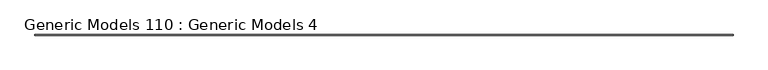
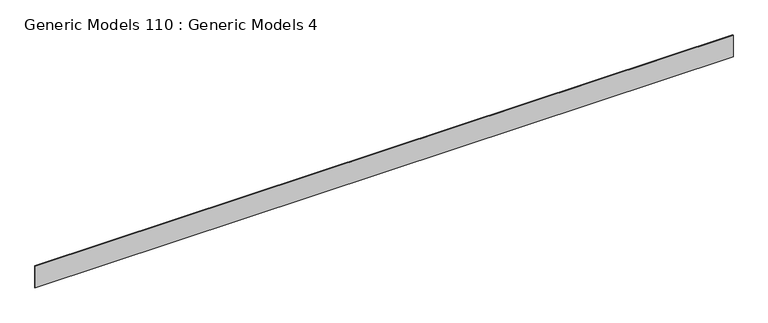
"""IFC4 building model written with IfcOpenShell, lengths in millimetres: proxy geometry, Generic Models 110 : Generic Models 4."""

from ifc_helpers import new_model, si_unit, frame, origin, place, context, project, spatial, polyline, outline, extrude, source, transform, mapped, element, save


def generic_models_110_generic_models_4_491da27e(model_context):
    return source(origin(), model_context, "Body", "SweptSolid", [
        extrude(outline(polyline([(8383.6828684, 7053.8569221), (8383.6828684, 7036.0769221), (-10259.9171316, 7036.0769221), (-10259.9171316, 7053.8569221), (8383.6828684, 7053.8569221)])), frame((0.0, 0.0, 125583.696), z_axis=(0.0, 0.0, 1.0), x_axis=(1.0, 0.0, 0.0)), (0.0, 0.0, 1.0), 609.6),
    ])


if __name__ == "__main__":
    model = new_model("IFC4")
    model_context = context("Model", 3, world=origin())
    ifc_project = project(units=[si_unit("LENGTHUNIT", "METRE", prefix="MILLI")], contexts=[model_context])
    site = spatial("IfcSite", under=ifc_project)
    building = spatial("IfcBuilding", under=site)
    placement = place(None, origin())
    generic_models_110_generic_models_4_shape = generic_models_110_generic_models_4_491da27e(model_context)
    element("IfcBuildingElementProxy", 1, Name="Generic Models 110 : Generic Models 4", ObjectType="Generic Models 110 : Generic Models 4", at=placement, inside=building, context=model_context, shape_type="MappedRepresentation", body=[
        mapped(generic_models_110_generic_models_4_shape, transform((0.0, 0.0, 0.0), x_axis=(1.0, 0.0, 0.0), y_axis=(0.0, 1.0, 0.0), z_axis=(0.0, 0.0, 1.0))),
    ])
    save(model, "model.ifc")

# Revit data of these elements
# Element 1 (IfcBuildingElementProxy, "Generic Models 110 : Generic Models 4")
#   Materials on its faces: "_7/8\" SMOOTH TROWEL INTERIOR STUCCO (COLOR PER OWNER)"
# Materials
#   "_7/8\" SMOOTH TROWEL INTERIOR STUCCO (COLOR PER OWNER)": class "Generic", colour RGB 233 233 233, transparency 0, Cost = 0
